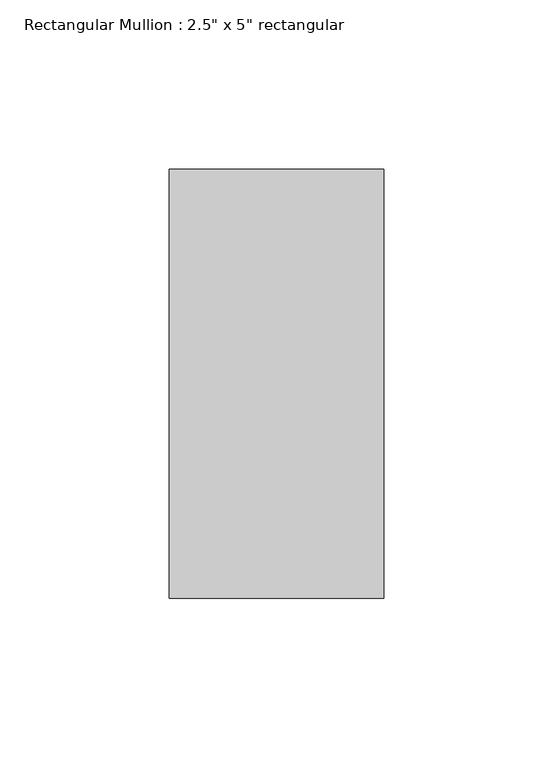
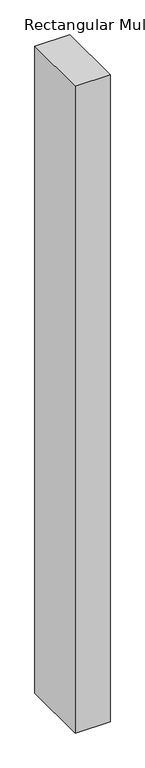
"""IFC4 building model written with IfcOpenShell, lengths in millimetres: member geometry."""

from ifc_helpers import new_model, si_unit, frame, origin, place, context, project, spatial, polyline, outline, extrude, source, transform, mapped, element, save


def member_c46932f7(model_context):
    return source(origin(), model_context, "Body", "SweptSolid", [
        extrude(outline(polyline([(31.75, 63.5), (31.75, -63.5), (-31.75, -63.5), (-31.75, 63.5), (31.75, 63.5)])), frame((0.0, 0.0, -1245.39375), z_axis=(0.0, 0.0, 1.0), x_axis=(1.0, 0.0, 0.0)), (0.0, 0.0, 1.0), 1245.39375),
    ])


if __name__ == "__main__":
    model = new_model("IFC4")
    model_context = context("Model", 3, world=origin())
    ifc_project = project(units=[si_unit("LENGTHUNIT", "METRE", prefix="MILLI")], contexts=[model_context])
    site = spatial("IfcSite", under=ifc_project)
    building = spatial("IfcBuilding", under=site)
    placement = place(None, origin())
    member_shape = member_c46932f7(model_context)
    element("IfcMember", 1, ObjectType="Rectangular Mullion : 2.5\" x 5\" rectangular", at=placement, inside=building, context=model_context, shape_type="MappedRepresentation", body=[
        mapped(member_shape, transform((0.0, 0.0, 0.0), x_axis=(1.0, 0.0, 0.0), y_axis=(0.0, 1.0, 0.0), z_axis=(0.0, 0.0, 1.0))),
    ])
    save(model, "model.ifc")

# Revit data of these elements
# Type "Rectangular Mullion : 2.5\" x 5\" rectangular"
#   built-in parameter 1007304 = 0.416667 (stored number, unit not read)
#   built-in parameter 1007301 = 0.104167 (stored number, unit not read)
#   built-in parameter 1007300 = 0.104167 (stored number, unit not read)
# Element 1 (IfcMember, "Rectangular Mullion : 2.5\" x 5\" rectangular")
#   Materials on its faces: "Metal - Aluminum"
# Materials
#   "Metal - Aluminum": class "Metal", colour RGB 140 140 140, transparency 0
